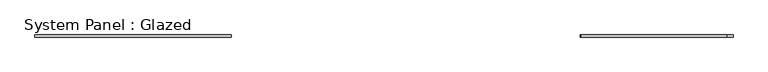
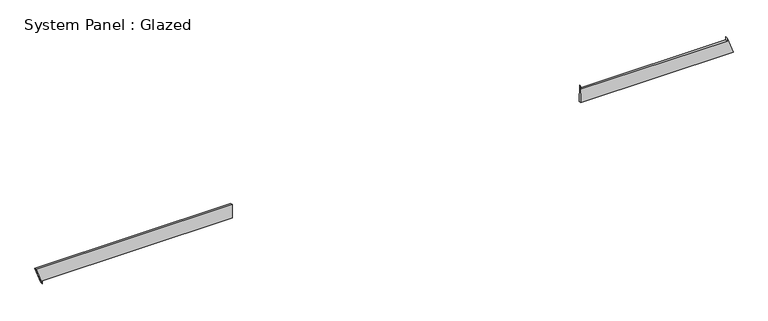
"""IFC4 building model written with IfcOpenShell, lengths in millimetres: plate geometry, System Panel : Glazed."""

import ifcopenshell
import ifcopenshell.guid

model = None  # the IFC model being written
_history = None  # IfcOwnerHistory: only IFC2X3 demands one
_inside = {}  # id of a spatial element -> (the spatial element, [elements in it])
_under = {}  # id of a project, library or spatial element -> (it, [spatial elements below it])
_declared = {}  # id of a project -> (the project, [libraries it declares])
_typed = {}  # id of a type object -> (the type object, [elements of that type])
_made_of = {}  # id of a material, layer set ... -> (it, [elements and type objects made of it])


def new_model(schema):
    """Start an empty IFC model of exactly this schema.

    Asked for "IFC4X3", IfcOpenShell would pick the latest addendum, in which some entities
    have other attributes; the version numbers below select the first issue.
    IFC2X3 requires an IfcOwnerHistory on every rooted entity: one is made here for all.
    """
    global model, _history
    if schema == "IFC4X3":
        model = ifcopenshell.file(schema_version=(4, 3, 0, 0))
    else:
        model = ifcopenshell.file(schema=schema)
    _inside.clear()
    _under.clear()
    _declared.clear()
    _typed.clear()
    _made_of.clear()
    _history = None
    if model.schema == "IFC2X3":
        org = make("IfcOrganization", Name="unknown")
        user = make(
            "IfcPersonAndOrganization",
            ThePerson=make("IfcPerson", FamilyName="unknown"),
            TheOrganization=org,
        )
        app = make(
            "IfcApplication",
            ApplicationDeveloper=org,
            Version="unknown",
            ApplicationFullName="unknown",
            ApplicationIdentifier="unknown",
        )
        _history = make(
            "IfcOwnerHistory",
            OwningUser=user,
            OwningApplication=app,
            ChangeAction="ADDED",
            CreationDate=0,
        )
    return model


def make(cls, **values):
    """One entity of the class cls with the attributes given. An attribute that is None is left unset."""
    return model.create_entity(
        cls, **{name: value for name, value in values.items() if value is not None}
    )


def rooted(cls, **values):
    """An entity with a GlobalId (a new one), such as an element, a storey or a relation."""
    return make(cls, GlobalId=ifcopenshell.guid.new(), OwnerHistory=_history, **values)


def si_unit(unit_type, name, prefix=None):
    """IfcSIUnit, for example si_unit("LENGTHUNIT", "METRE", prefix="MILLI")."""
    return make("IfcSIUnit", UnitType=unit_type, Prefix=prefix, Name=name)


def assignment(units):
    """IfcUnitAssignment: the units of a project."""
    return None if units is None else make("IfcUnitAssignment", Units=units)


def point(xyz):
    """IfcCartesianPoint."""
    return None if xyz is None else make("IfcCartesianPoint", Coordinates=xyz)


def direction(xyz):
    """IfcDirection."""
    return None if xyz is None else make("IfcDirection", DirectionRatios=xyz)


def frame(location, z_axis=None, x_axis=None):
    """IfcAxis2Placement3D, a coordinate frame: its origin and axes. An axis left out is left unset."""
    return make(
        "IfcAxis2Placement3D",
        Location=point(location),
        Axis=direction(z_axis),
        RefDirection=direction(x_axis),
    )


def origin():
    """The frame at (0, 0, 0) with its axes left unset."""
    return frame((0.0, 0.0, 0.0))


def place(relative_to, where):
    """IfcLocalPlacement: puts the frame where relative to a parent placement (None: the world)."""
    return make(
        "IfcLocalPlacement", PlacementRelTo=relative_to, RelativePlacement=where
    )


def context(
    kind, dimensions, precision=None, world=None, true_north=None, identifier=None
):
    """IfcGeometricRepresentationContext, for example the 3D "Model" context."""
    return make(
        "IfcGeometricRepresentationContext",
        ContextIdentifier=identifier,
        ContextType=kind,
        CoordinateSpaceDimension=dimensions,
        Precision=precision,
        WorldCoordinateSystem=world,
        TrueNorth=true_north,
    )


def project(units=None, contexts=None):
    """IfcProject with its units and contexts."""
    return rooted(
        "IfcProject",
        Name="project",
        RepresentationContexts=contexts,
        UnitsInContext=assignment(units),
    )


def spatial(cls, under=None, at=None, **own):
    """A site, building, storey or space (cls), placed at a placement, below another one or the project."""
    s = rooted(cls, ObjectPlacement=at, **own)
    if under is not None:
        _under.setdefault(under.id(), (under, []))[1].append(s)
    return s


def polyline(points):
    """IfcPolyline through the points."""
    return make("IfcPolyline", Points=[point(p) for p in points])


def outline(outer, holes=None, kind="AREA"):
    """IfcArbitraryClosedProfileDef: a profile drawn as a closed curve; with holes, ...WithVoids."""
    if holes is None:
        return make("IfcArbitraryClosedProfileDef", ProfileType=kind, OuterCurve=outer)
    return make(
        "IfcArbitraryProfileDefWithVoids",
        ProfileType=kind,
        OuterCurve=outer,
        InnerCurves=holes,
    )


def extrude(swept, where, along, depth):
    """IfcExtrudedAreaSolid: the profile swept, set in the frame where, extruded along a direction by depth."""
    return make(
        "IfcExtrudedAreaSolid",
        SweptArea=swept,
        Position=where,
        ExtrudedDirection=direction(along),
        Depth=depth,
    )


def shape(context_of_items, identifier, shape_type, items):
    """IfcShapeRepresentation: the items that make up one representation, for example the "Body"."""
    return make(
        "IfcShapeRepresentation",
        ContextOfItems=context_of_items,
        RepresentationIdentifier=identifier,
        RepresentationType=shape_type,
        Items=items,
    )


def source(mapping_origin, context_of_items, identifier, shape_type, items):
    """IfcRepresentationMap: a shape defined once, which mapped items show again and again."""
    return make(
        "IfcRepresentationMap",
        MappingOrigin=mapping_origin,
        MappedRepresentation=shape(context_of_items, identifier, shape_type, items),
    )


def transform(
    local_origin,
    x_axis=None,
    y_axis=None,
    z_axis=None,
    scale=None,
    scale2=None,
    scale3=None,
    uniform=True,
):
    """IfcCartesianTransformationOperator3D, or its non-uniform kind. x_axis, y_axis, z_axis: its Axis1, 2, 3."""
    if uniform:
        return make(
            "IfcCartesianTransformationOperator3D",
            Axis1=direction(x_axis),
            Axis2=direction(y_axis),
            LocalOrigin=point(local_origin),
            Scale=scale,
            Axis3=direction(z_axis),
        )
    return make(
        "IfcCartesianTransformationOperator3DnonUniform",
        Axis1=direction(x_axis),
        Axis2=direction(y_axis),
        LocalOrigin=point(local_origin),
        Scale=scale,
        Axis3=direction(z_axis),
        Scale2=scale2,
        Scale3=scale3,
    )


def mapped(mapping_source, mapping_target):
    """IfcMappedItem: shows the shape of a source again, moved by a transform."""
    return make(
        "IfcMappedItem", MappingSource=mapping_source, MappingTarget=mapping_target
    )


def made_of(thing, what):
    """Note that an element or type object is made of a material, layer set ...; save() writes the relation."""
    if what is not None:
        _made_of.setdefault(what.id(), (what, []))[1].append(thing)
    return thing


def element(
    cls,
    number,
    at=None,
    inside=None,
    cuts=None,
    type_object=None,
    material=None,
    context=None,
    identifier="Body",
    shape_type=None,
    held_by="IfcProductDefinitionShape",
    body=None,
    shapes=None,
    **own,
):
    """One element of the class cls, such as IfcWall. Its Tag is "e" and its number.

    at: its placement. inside: the storey or other place that contains it. cuts: it is an
    opening in that element (IfcRelVoidsElement). A single representation is given by context,
    identifier, shape_type and body (its items); several are given by shapes. held_by: the class
    of the entity that holds the representations. save() writes the other relations.
    """
    e = rooted(cls, Tag="e%d" % number, ObjectPlacement=at, **own)
    if body is not None:
        shapes = [shape(context, identifier, shape_type, body)]
    if shapes is not None:
        e.Representation = make(held_by, Representations=shapes)
    if inside is not None:
        _inside.setdefault(inside.id(), (inside, []))[1].append(e)
    if cuts is not None:
        rooted(
            "IfcRelVoidsElement", RelatingBuildingElement=cuts, RelatedOpeningElement=e
        )
    if type_object is not None:
        _typed.setdefault(type_object.id(), (type_object, []))[1].append(e)
    return made_of(e, material)


def aggregate(whole, parts):
    """IfcRelAggregates: a whole, such as a stair, and the parts it consists of."""
    return rooted("IfcRelAggregates", RelatingObject=whole, RelatedObjects=parts)


def save(model, path):
    """Write the relations noted so far, then the file.

    IfcRelAggregates (storeys below a building ...), IfcRelContainedInSpatialStructure (elements
    in a storey), IfcRelDefinesByType, IfcRelAssociatesMaterial and IfcRelDeclares: one each for
    every whole, place, type object, material and project.
    """
    for whole, parts in _under.values():
        aggregate(whole, parts)
    for where, things in _inside.values():
        rooted(
            "IfcRelContainedInSpatialStructure",
            RelatedElements=things,
            RelatingStructure=where,
        )
    for kind, things in _typed.values():
        rooted("IfcRelDefinesByType", RelatedObjects=things, RelatingType=kind)
    for what, things in _made_of.values():
        rooted("IfcRelAssociatesMaterial", RelatedObjects=things, RelatingMaterial=what)
    for by, libraries in _declared.values():
        rooted("IfcRelDeclares", RelatingContext=by, RelatedDefinitions=libraries)
    model.write(path)


def system_panel_glazed_0fd24995(model_context):
    return source(origin(), model_context, "Body", "SweptSolid", [
        extrude(outline(polyline([(0.0, -3957.0720499), (35.3553391, -3957.0720499), (35.3553391, -1759.4448109), (198.9258324, -1762.342403), (198.9069288, -4026.9181807), (0.0, -3957.0720499)])), frame((0.0, -49.5, 0.0), z_axis=(0.0, 1.0, 0.0), x_axis=(0.0, 0.0, 1.0)), (0.0, 0.0, 1.0), 25.0),
        extrude(outline(polyline([(35.3553391, 2263.6353155), (35.3553391, 4026.9181807), (234.328916, 3957.2301733), (198.9735769, 3957.2304684), (198.9594776, 2268.1982411), (234.3148167, 2268.197946), (35.3553391, 2263.6353155)])), frame((0.0, -49.5, 0.0), z_axis=(0.0, 1.0, 0.0), x_axis=(0.0, 0.0, 1.0)), (0.0, 0.0, 1.0), 25.0),
    ])


if __name__ == "__main__":
    model = new_model("IFC4")
    model_context = context("Model", 3, world=origin())
    ifc_project = project(units=[si_unit("LENGTHUNIT", "METRE", prefix="MILLI")], contexts=[model_context])
    site = spatial("IfcSite", under=ifc_project)
    building = spatial("IfcBuilding", under=site)
    placement = place(None, origin())
    system_panel_glazed_shape = system_panel_glazed_0fd24995(model_context)
    element("IfcPlate", 1, ObjectType="System Panel : Glazed", at=placement, inside=building, context=model_context, shape_type="MappedRepresentation", body=[
        mapped(system_panel_glazed_shape, transform((0.0, 0.0, 0.0), x_axis=(1.0, 0.0, 0.0), y_axis=(0.0, 1.0, 0.0), z_axis=(0.0, 0.0, 1.0))),
    ])
    save(model, "model.ifc")

# Revit data of these elements
# Element 1 (IfcPlate, "System Panel : Glazed")
#   Materials on its faces: "Glass"
# Materials
#   "Glass": class "Glass", colour RGB 218 227 224, transparency 0.85, Description = "Soda Lime Glass", Cost = 0
